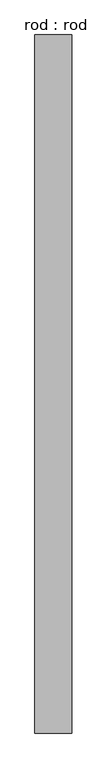
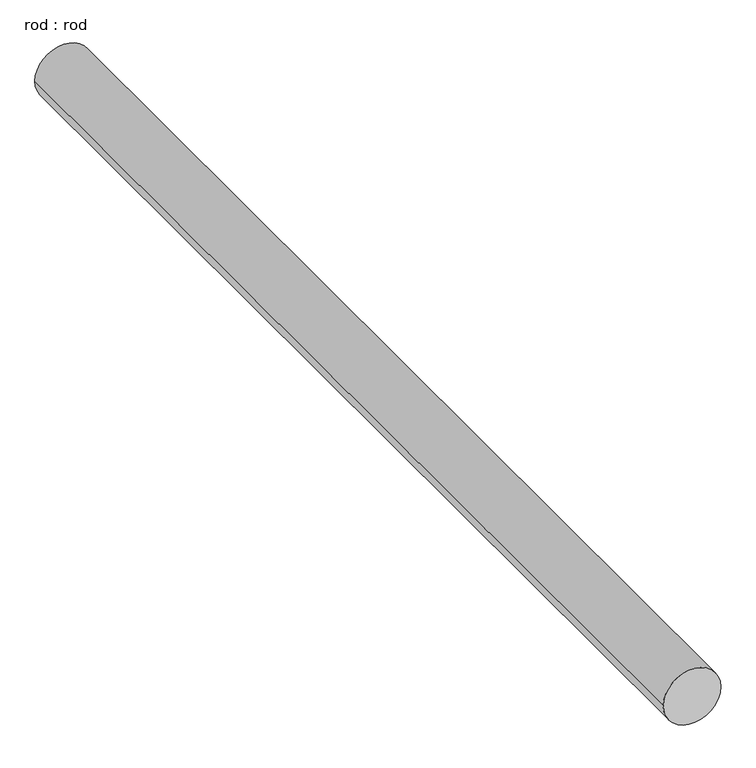
"""IFC4 building model written with IfcOpenShell, lengths in millimetres: proxy geometry, rod : rod."""

from ifc_helpers import new_model, si_unit, point, frame, frame_2d, origin, place, context, project, spatial, circle_curve, trimmed, segment, composite_curve, outline, extrude, source, transform, mapped, element, save


def rod_rod_e3e6feec(model_context):
    return source(origin(), model_context, "Body", "SweptSolid", [
        extrude(outline(composite_curve([segment(trimmed(circle_curve(frame_2d((0.0108462, 0.0)), 200.0), [point((0.0108462, 200.0))], [point((0.0108462, -200.0))], False, "CARTESIAN"), True, "CONTINUOUS"), segment(trimmed(circle_curve(frame_2d((0.0108462, 0.0)), 200.0), [point((0.0108462, -200.0))], [point((0.0108462, 200.0))], False, "CARTESIAN"), True, "CONTINUOUS")], self_intersect=False)), frame((0.0, 310.1905104, 0.0), z_axis=(0.0, 1.0, 0.0), x_axis=(0.0, 0.0, 1.0)), (0.0, 0.0, 1.0), 7565.0762099),
    ])


if __name__ == "__main__":
    model = new_model("IFC4")
    model_context = context("Model", 3, world=origin())
    ifc_project = project(units=[si_unit("LENGTHUNIT", "METRE", prefix="MILLI")], contexts=[model_context])
    site = spatial("IfcSite", under=ifc_project)
    building = spatial("IfcBuilding", under=site)
    placement = place(None, origin())
    rod_rod_shape = rod_rod_e3e6feec(model_context)
    element("IfcBuildingElementProxy", 1, Name="rod : rod", ObjectType="rod : rod", at=placement, inside=building, context=model_context, shape_type="MappedRepresentation", body=[
        mapped(rod_rod_shape, transform((0.0, 0.0, 0.0), x_axis=(1.0, 0.0, 0.0), y_axis=(0.0, 1.0, 0.0), z_axis=(0.0, 0.0, 1.0))),
    ])
    save(model, "model.ifc")

# Revit data of these elements
# Type "rod : rod"
#   Default Elevation = 0
